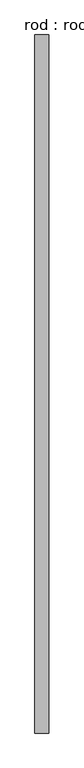
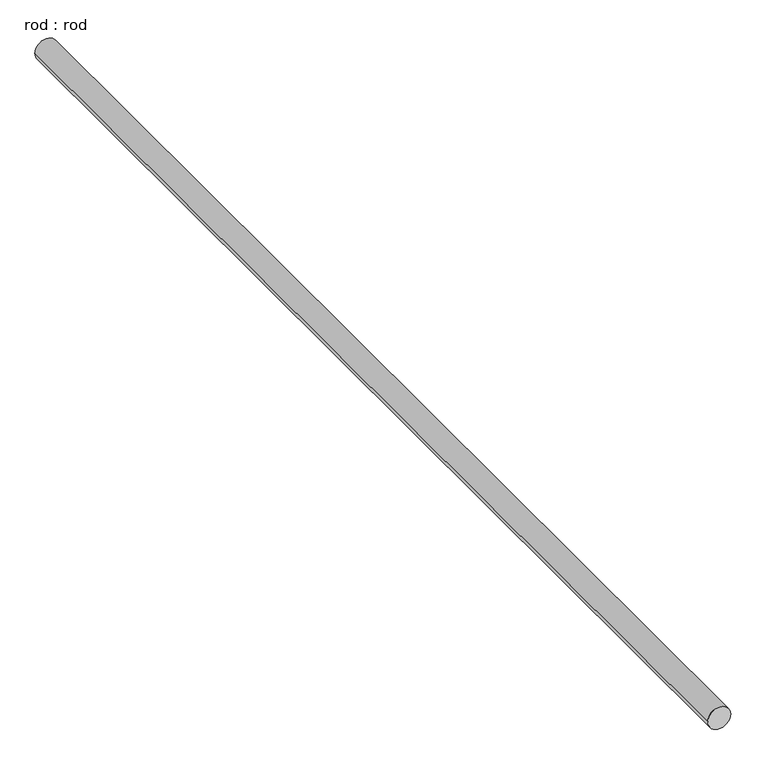
"""IFC4 building model written with IfcOpenShell, lengths in millimetres: proxy geometry, rod : rod."""

from ifc_helpers import new_model, si_unit, point, frame, frame_2d, origin, place, context, project, spatial, circle_curve, trimmed, segment, composite_curve, outline, extrude, source, transform, mapped, element, save


def rod_rod_d2c854aa(model_context):
    return source(origin(), model_context, "Body", "SweptSolid", [
        extrude(outline(composite_curve([segment(trimmed(circle_curve(frame_2d((0.0108462, 0.0)), 200.0), [point((0.0108462, 200.0))], [point((0.0108462, -200.0))], False, "CARTESIAN"), True, "CONTINUOUS"), segment(trimmed(circle_curve(frame_2d((0.0108462, 0.0)), 200.0), [point((0.0108462, -200.0))], [point((0.0108462, 200.0))], False, "CARTESIAN"), True, "CONTINUOUS")], self_intersect=False)), frame((0.0, -6074.9023925, 0.0), z_axis=(0.0, 1.0, 0.0), x_axis=(0.0, 0.0, 1.0)), (0.0, 0.0, 1.0), 20335.2620158),
    ])


if __name__ == "__main__":
    model = new_model("IFC4")
    model_context = context("Model", 3, world=origin())
    ifc_project = project(units=[si_unit("LENGTHUNIT", "METRE", prefix="MILLI")], contexts=[model_context])
    site = spatial("IfcSite", under=ifc_project)
    building = spatial("IfcBuilding", under=site)
    placement = place(None, origin())
    rod_rod_shape = rod_rod_d2c854aa(model_context)
    element("IfcBuildingElementProxy", 1, Name="rod : rod", ObjectType="rod : rod", at=placement, inside=building, context=model_context, shape_type="MappedRepresentation", body=[
        mapped(rod_rod_shape, transform((0.0, 0.0, 0.0), x_axis=(1.0, 0.0, 0.0), y_axis=(0.0, 1.0, 0.0), z_axis=(0.0, 0.0, 1.0))),
    ])
    save(model, "model.ifc")

# Revit data of these elements
# Type "rod : rod"
#   Default Elevation = 0
